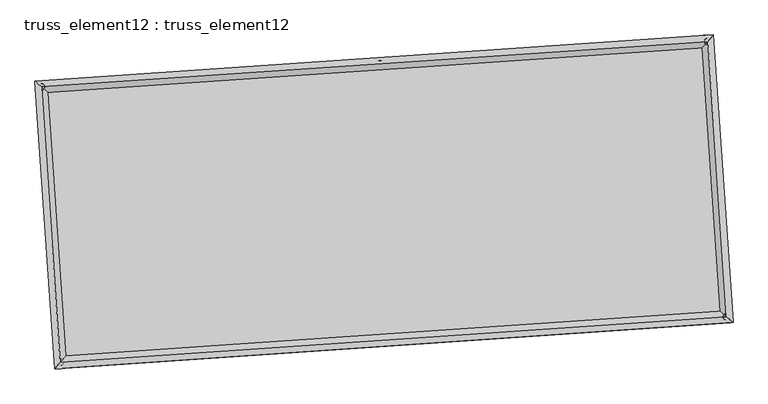
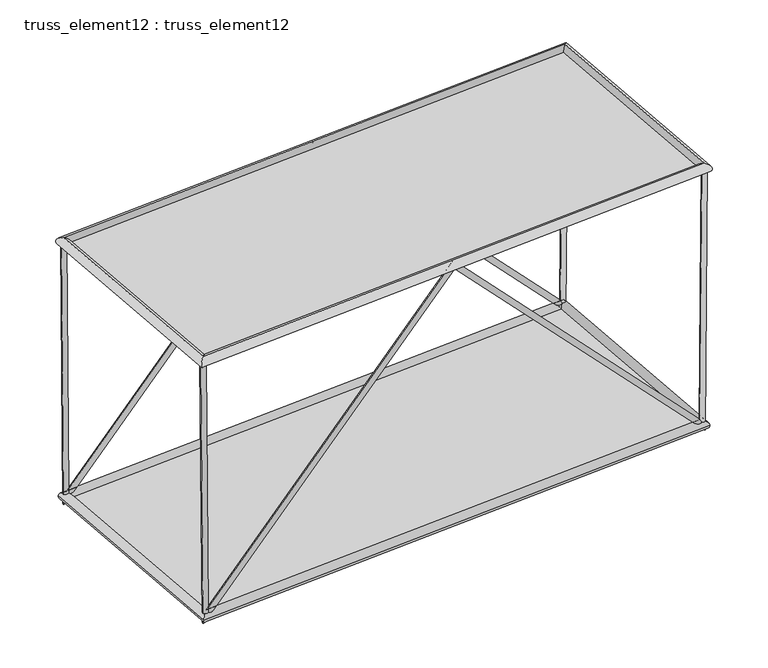
"""IFC4 building model written with IfcOpenShell, lengths in millimetres: plate geometry, truss_element12 : truss_element12."""

from ifc_helpers import new_model, si_unit, frame, origin, origin_with_axes, place, context, project, spatial, polyline, circle_curve, ellipse_curve, outline, extrude, source, transform, mapped, element, save
from ifc_brep_helpers import plane_surface, cylinder_surface, advanced_brep


def truss_element12_truss_element12_5f5549ff(model_context):
    return source(origin(), model_context, "Body", "SolidModel", [
        advanced_brep(
        [(-3707.9964238, 2273.2882323, 5000.2443705), (-3807.096081, 2259.9272328, 4999.3831901), (-3665.9998224, 2276.1518209, 123.0904436), (-3762.9870604, 2262.9348592, -123.0904436), (1064.0881488, 2598.6785389, 5071.9331188), (1064.5308451, 2592.1049541, 4927.688056), (5793.4565797, 2921.1561942, 123.0852691), (5891.3043973, 2921.2242943, -123.0852691), (5836.1672791, 2924.0684744, 5000.2453052), (5936.1632135, 2924.2830465, 4999.3694838)],
        [
            (0, 1, circle_curve(frame((-3757.5462524, 2266.6077325, 4999.8137803), z_axis=(-0.008610562197328881, -0.0005871215044246289, 0.9999627560599369), x_axis=(-0.13361007490078702, 0.9910338160498287, -0.0005686217728233661)), 50.0)),
            (1, 0, circle_curve(frame((-3757.5462524, 2266.6077325, 4999.8137803), z_axis=(-0.008610562197328881, -0.0005871215044246289, 0.9999627560599369), x_axis=(-0.13361007490078702, 0.9910338160498287, -0.0005686217728233661)), 50.0)),
            (0, 2),
            (2, 3, ellipse_curve(frame((-3714.4934414, 2269.54334, 0.0), z_axis=(-0.9273750844968209, -0.06323418172910877, 0.3687504453089708), x_axis=(0.36789619657997696, 0.02508544314041891, 0.9295284337148788)), 132.7108104, 50.0)),
            (3, 1),
            (3, 2, ellipse_curve(frame((-3714.4934414, 2269.54334, 0.0), z_axis=(-0.9273750844968209, -0.06323418172910877, 0.3687504453089708), x_axis=(0.36789619657997696, 0.02508544314041891, 0.9295284337148788)), 132.7108104, 50.0)),
            (2, 4),
            (4, 5, ellipse_curve(frame((1064.309497, 2595.3917465, 4999.8105874), z_axis=(-0.9976833953446986, -0.06802823817891461, 3.825893912910826e-05), x_axis=(-3.817030832084868e-05, -2.6026882256253026e-06, -0.9999999992681269)), 72.2795775, 50.0)),
            (5, 3),
            (5, 4, ellipse_curve(frame((1064.309497, 2595.3917465, 4999.8105874), z_axis=(-0.9976833953446986, -0.06802823817891461, 3.825893912910826e-05), x_axis=(-3.817030832084868e-05, -2.6026882256253026e-06, -0.9999999992681269)), 72.2795775, 50.0)),
            (4, 6),
            (6, 7, ellipse_curve(frame((5842.3804885, 2921.1902443, 0.0), z_axis=(-0.9274161456323363, -0.06323698153185128, -0.3686466831360366), x_axis=(-0.3677926747828999, -0.025078384382599298, 0.9295695901936544)), 132.6993561, 50.0)),
            (7, 5),
            (7, 6, ellipse_curve(frame((5842.3804885, 2921.1902443, 0.0), z_axis=(-0.9274161456323363, -0.06323698153185128, -0.3686466831360366), x_axis=(-0.3677926747828999, -0.025078384382599298, 0.9295695901936544)), 132.6993561, 50.0)),
            (8, 9, circle_curve(frame((5886.1652463, 2924.1757604, 4999.8073945), z_axis=(0.00875695156738284, 0.0005971032390905219, 0.9999614788915463), x_axis=(-0.002150867604689313, 0.9999975196721189, -0.0005782889909695317)), 50.0)),
            (9, 8, circle_curve(frame((5886.1652463, 2924.1757604, 4999.8073945), z_axis=(0.00875695156738284, 0.0005971032390905219, 0.9999614788915463), x_axis=(-0.002150867604689313, 0.9999975196721189, -0.0005782889909695317)), 50.0)),
            (6, 8),
            (9, 7),
        ],
        [
            plane_surface(frame((-3757.5462524, 2316.6077239, 4999.8431375), z_axis=(-0.008610562197328035, -0.0005871215044280537, 0.9999627560599371), x_axis=(0.999962928422172, -5.055633651274154e-06, 0.008610560713137268))),
            cylinder_surface(frame((-3757.5462524, 2266.6077325, 4999.8137803), z_axis=(-0.008610562197328883, -0.000587121504424629, 0.9999627560599371), x_axis=(-0.13361007490078702, 0.9910338160498287, -0.0005686217728233661)), 50.0),
            cylinder_surface(frame((-3714.4934414, 2269.54334, 0.0), z_axis=(-0.6901833653788351, -0.04706098005258923, -0.7221026148068121), x_axis=(-0.02041511250677689, 0.9987521502411405, -0.04557812600397415)), 50.0),
            cylinder_surface(frame((1064.309497, 2595.3917465, 4999.8105874), z_axis=(-0.6901282375994761, -0.047057221098874814, 0.7221555466866489), x_axis=(-0.11534922537103473, 0.9922789539632748, -0.045574485491901566)), 50.0),
            plane_surface(frame((5886.1652463, 2874.1757694, 4999.8372508), z_axis=(0.00875695156738239, 0.0005971032390901972, 0.9999614788915465), x_axis=(0.9999616571645369, -5.2290046408387525e-06, -0.008756950006194586))),
            cylinder_surface(frame((5842.3804885, 2921.1902443, 0.0), z_axis=(-0.00875695156738284, -0.0005971032390905219, -0.9999614788915463), x_axis=(-0.002150867604689313, 0.9999975196721189, -0.0005782889909695317)), 50.0),
        ],
        [
            (0, [[1, 2]]),
            (1, [[-1, 3, 4, 5]]),
            (1, [[-2, -5, 6, -3]]),
            (2, [[-4, 7, 8, 9]]),
            (2, [[-6, -9, 10, -7]]),
            (3, [[-8, 11, 12, 13]]),
            (3, [[-10, -13, 14, -11]]),
            (4, [[15, 16]]),
            (5, [[-12, 17, -16, 18]]),
            (5, [[-14, -18, -15, -17]]),
        ],
    ),
        advanced_brep(
        [(-3435.8834709, -1717.445352, 5000.2443705), (-3534.9831281, -1730.8063515, 4999.3831901), (-3393.8868695, -1714.5817634, 123.0904436), (-3490.8741075, -1727.7987251, -123.0904436), (1336.2011017, -1392.0550454, 5071.9331188), (1336.643798, -1398.6286302, 4927.688056), (6065.5695326, -1069.5773901, 123.0852691), (6163.4173503, -1069.50929, -123.0852691), (6108.2802321, -1066.6651099, 5000.2453052), (6208.2761665, -1066.4505378, 4999.3694838)],
        [
            (0, 1, circle_curve(frame((-3485.4332995, -1724.1258518, 4999.8137803), z_axis=(-0.008610562197328883, -0.0005871215044246118, 0.9999627560599369), x_axis=(-0.13361007490078664, 0.9910338160498287, -0.0005686217728233801)), 50.0)),
            (1, 0, circle_curve(frame((-3485.4332995, -1724.1258518, 4999.8137803), z_axis=(-0.008610562197328883, -0.0005871215044246118, 0.9999627560599369), x_axis=(-0.13361007490078664, 0.9910338160498287, -0.0005686217728233801)), 50.0)),
            (0, 2),
            (2, 3, ellipse_curve(frame((-3442.3804885, -1721.1902443, 0.0), z_axis=(-0.9273750844968209, -0.06323418172910855, 0.3687504453089707), x_axis=(0.3678961965799769, 0.025085443140418835, 0.9295284337148788)), 132.7108104, 50.0)),
            (3, 1),
            (3, 2, ellipse_curve(frame((-3442.3804885, -1721.1902443, 0.0), z_axis=(-0.9273750844968209, -0.06323418172910855, 0.3687504453089707), x_axis=(0.3678961965799769, 0.025085443140418835, 0.9295284337148788)), 132.7108104, 50.0)),
            (2, 4),
            (4, 5, ellipse_curve(frame((1336.4224499, -1395.3418378, 4999.8105874), z_axis=(-0.9976833953446986, -0.06802823817891454, 3.825893912894776e-05), x_axis=(-3.817030832069493e-05, -2.6026882254811685e-06, -0.9999999992681269)), 72.2795775, 50.0)),
            (5, 3),
            (5, 4, ellipse_curve(frame((1336.4224499, -1395.3418378, 4999.8105874), z_axis=(-0.9976833953446986, -0.06802823817891454, 3.825893912894776e-05), x_axis=(-3.817030832069493e-05, -2.6026882254811685e-06, -0.9999999992681269)), 72.2795775, 50.0)),
            (4, 6),
            (6, 7, ellipse_curve(frame((6114.4934414, -1069.54334, 0.0), z_axis=(-0.9274161456323362, -0.06323698153185144, -0.3686466831360369), x_axis=(-0.36779267478290023, -0.025078384382599305, 0.9295695901936543)), 132.6993561, 50.0)),
            (7, 5),
            (7, 6, ellipse_curve(frame((6114.4934414, -1069.54334, 0.0), z_axis=(-0.9274161456323362, -0.06323698153185144, -0.3686466831360369), x_axis=(-0.36779267478290023, -0.025078384382599305, 0.9295695901936543)), 132.6993561, 50.0)),
            (8, 9, circle_curve(frame((6158.2781993, -1066.5578239, 4999.8073945), z_axis=(0.00875695156738245, 0.0005971032390905659, 0.9999614788915463), x_axis=(-0.002150867604689674, 0.999997519672119, -0.0005782889909695735)), 50.0)),
            (9, 8, circle_curve(frame((6158.2781993, -1066.5578239, 4999.8073945), z_axis=(0.00875695156738245, 0.0005971032390905659, 0.9999614788915463), x_axis=(-0.002150867604689674, 0.999997519672119, -0.0005782889909695735)), 50.0)),
            (6, 8),
            (9, 7),
        ],
        [
            plane_surface(frame((-3485.4332995, -1674.1258604, 4999.8431375), z_axis=(-0.008610562197328035, -0.0005871215044280489, 0.9999627560599371), x_axis=(0.999962928422172, -5.055633651274154e-06, 0.008610560713137268))),
            cylinder_surface(frame((-3485.4332995, -1724.1258518, 4999.8137803), z_axis=(-0.008610562197328885, -0.0005871215044246119, 0.9999627560599371), x_axis=(-0.13361007490078664, 0.9910338160498287, -0.0005686217728233801)), 50.0),
            cylinder_surface(frame((-3442.3804885, -1721.1902443, 0.0), z_axis=(-0.690183365378835, -0.047060980052589074, -0.7221026148068123), x_axis=(-0.02041511250677676, 0.9987521502411404, -0.045578126003974054)), 50.0),
            cylinder_surface(frame((1336.4224499, -1395.3418378, 4999.8105874), z_axis=(-0.6901282375994762, -0.04705722109887487, 0.7221555466866488), x_axis=(-0.11534922537103474, 0.9922789539632748, -0.045574485491901524)), 50.0),
            plane_surface(frame((6158.2781993, -1116.5578149, 4999.8372508), z_axis=(0.00875695156738239, 0.0005971032390901939, 0.9999614788915465), x_axis=(0.9999616571645369, -5.229004640394663e-06, -0.008756950006194586))),
            cylinder_surface(frame((6114.4934414, -1069.54334, 0.0), z_axis=(-0.00875695156738245, -0.0005971032390905659, -0.9999614788915463), x_axis=(-0.002150867604689674, 0.999997519672119, -0.0005782889909695735)), 50.0),
        ],
        [
            (0, [[1, 2]]),
            (1, [[-1, 3, 4, 5]]),
            (1, [[-2, -5, 6, -3]]),
            (2, [[-4, 7, 8, 9]]),
            (2, [[-6, -9, 10, -7]]),
            (3, [[-8, 11, 12, 13]]),
            (3, [[-10, -13, 14, -11]]),
            (4, [[15, 16]]),
            (5, [[-12, 17, -16, 18]]),
            (5, [[-14, -18, -15, -17]]),
        ],
    ),
        advanced_brep(
        [(-3485.434982, -1724.1277166, 4909.8137803), (-3485.431617, -1724.123987, 5089.8137803), (-3757.5443323, 2266.6061134, 5089.8137803), (-3757.5481725, 2266.6093517, 4909.8137803), (5886.1636825, 2924.1739037, 5089.8073944), (5886.1668102, 2924.1776171, 4909.8073945), (6158.2763978, -1066.5561966, 5089.8073944), (6158.2800007, -1066.5594511, 4909.8073945)],
        [
            (0, 1, ellipse_curve(frame((-3485.4332995, -1724.1258518, 4999.8137803), z_axis=(-0.7535719234053024, 0.6573654662780931, 4.6714499693675804e-07), x_axis=(-0.6573654662779286, -0.753571923405446, 4.6714499693680886e-07)), 127.2792206, 90.0)),
            (1, 2),
            (2, 3, ellipse_curve(frame((-3757.5462524, 2266.6077325, 4999.8137803), z_axis=(-0.6573654662779286, -0.753571923405446, 4.6714499693685635e-07), x_axis=(0.7535719234053025, -0.657365466278093, -4.6714499693680563e-07)), 127.2792206, 90.0)),
            (3, 0),
            (1, 0, ellipse_curve(frame((-3485.4332995, -1724.1258518, 4999.8137803), z_axis=(-0.7535719234053024, 0.6573654662780931, 4.6714499693675804e-07), x_axis=(-0.6573654662779286, -0.753571923405446, 4.6714499693680886e-07)), 127.2792206, 90.0)),
            (3, 2, ellipse_curve(frame((-3757.5462524, 2266.6077325, 4999.8137803), z_axis=(-0.6573654662779286, -0.753571923405446, 4.6714499693685635e-07), x_axis=(0.7535719234053025, -0.657365466278093, -4.6714499693680563e-07)), 127.2792206, 90.0)),
            (2, 4),
            (4, 5, ellipse_curve(frame((5886.1652463, 2924.1757604, 4999.8073945), z_axis=(-0.7535719234053022, 0.6573654662780931, 4.671449969368529e-07), x_axis=(-0.657365466277929, -0.7535719234054455, 4.6714499693680907e-07)), 127.2792206, 90.0)),
            (5, 3),
            (5, 4, ellipse_curve(frame((5886.1652463, 2924.1757604, 4999.8073945), z_axis=(-0.7535719234053022, 0.6573654662780931, 4.671449969368529e-07), x_axis=(-0.657365466277929, -0.7535719234054455, 4.6714499693680907e-07)), 127.2792206, 90.0)),
            (4, 6),
            (6, 7, ellipse_curve(frame((6158.2781993, -1066.5578239, 4999.8073945), z_axis=(0.6573654662779289, 0.7535719234054455, -4.671449969367615e-07), x_axis=(-0.7535719234053019, 0.6573654662780936, 4.671449969368051e-07)), 127.2792206, 90.0)),
            (7, 5),
            (7, 6, ellipse_curve(frame((6158.2781993, -1066.5578239, 4999.8073945), z_axis=(0.6573654662779289, 0.7535719234054455, -4.671449969367615e-07), x_axis=(-0.7535719234053019, 0.6573654662780936, 4.671449969368051e-07)), 127.2792206, 90.0)),
            (6, 1),
            (0, 7),
        ],
        [
            cylinder_surface(frame((-3485.4332995, -1724.1258518, 4999.8137803), z_axis=(0.06802823822869912, -0.9976833960748768, 0.0), x_axis=(-0.997683395874126, -0.0680282382150107, 2.0060750261440357e-05)), 90.0),
            cylinder_surface(frame((-3757.5462524, 2266.6077325, 4999.8137803), z_axis=(-0.9976833960746592, -0.06802823822868387, 6.606427902628043e-07), x_axis=(-0.06802823820311017, 0.9976833958880026, 1.9400107471301905e-05)), 90.0),
            cylinder_surface(frame((5886.1652463, 2924.1757604, 4999.8073945), z_axis=(-0.06802823822869865, 0.997683396074877, 0.0), x_axis=(0.9976833958996999, 0.068028238216754, 1.873946468116346e-05)), 90.0),
            cylinder_surface(frame((6158.2781993, -1066.5578239, 4999.8073945), z_axis=(0.9976833960746592, 0.06802823822868365, -6.606427902627372e-07), x_axis=(0.06802823822868365, -0.9976833958862589, 1.9400107471301912e-05)), 90.0),
        ],
        [
            (0, [[1, 2, 3, 4]]),
            (0, [[5, -4, 6, -2]]),
            (1, [[-3, 7, 8, 9]]),
            (1, [[-6, -9, 10, -7]]),
            (2, [[-8, 11, 12, 13]]),
            (2, [[-10, -13, 14, -11]]),
            (3, [[-12, 15, -1, 16]]),
            (3, [[-14, -16, -5, -15]]),
        ],
    ),
        advanced_brep(
        [(-3358.7115243, -1625.2761972, 0.0), (-3526.0494527, -1817.1042913, 0.0), (-3810.4074885, 2353.2123043, 0.0), (-3618.5793943, 2185.8743758, 0.0), (5926.0494527, 3017.1042913, 0.0), (5758.7115243, 2825.2761972, 0.0), (6210.4074885, -1153.2123043, 0.0), (6018.5793943, -985.8743758, 0.0)],
        [
            (0, 1, ellipse_curve(frame((-3442.3804885, -1721.1902443, 0.0), z_axis=(-0.753571923405459, 0.6573654662780796, 0.0), x_axis=(-0.6573654662780796, -0.753571923405459, 0.0)), 127.2792206, 90.0)),
            (1, 2),
            (2, 3, ellipse_curve(frame((-3714.4934414, 2269.54334, 0.0), z_axis=(-0.6573654662780796, -0.753571923405459, 0.0), x_axis=(0.753571923405459, -0.6573654662780796, 0.0)), 127.2792206, 90.0)),
            (3, 0),
            (1, 0, ellipse_curve(frame((-3442.3804885, -1721.1902443, 0.0), z_axis=(-0.753571923405459, 0.6573654662780796, 0.0), x_axis=(-0.6573654662780796, -0.753571923405459, 0.0)), 127.2792206, 90.0)),
            (3, 2, ellipse_curve(frame((-3714.4934414, 2269.54334, 0.0), z_axis=(-0.6573654662780796, -0.753571923405459, 0.0), x_axis=(0.753571923405459, -0.6573654662780796, 0.0)), 127.2792206, 90.0)),
            (2, 4),
            (4, 5, ellipse_curve(frame((5842.3804885, 2921.1902443, 0.0), z_axis=(-0.7535719234054589, 0.6573654662780797, 0.0), x_axis=(-0.6573654662780798, -0.7535719234054588, 0.0)), 127.2792206, 90.0)),
            (5, 3),
            (5, 4, ellipse_curve(frame((5842.3804885, 2921.1902443, 0.0), z_axis=(-0.7535719234054589, 0.6573654662780797, 0.0), x_axis=(-0.6573654662780798, -0.7535719234054588, 0.0)), 127.2792206, 90.0)),
            (4, 6),
            (6, 7, ellipse_curve(frame((6114.4934414, -1069.54334, 0.0), z_axis=(0.6573654662780797, 0.7535719234054589, 0.0), x_axis=(-0.7535719234054589, 0.6573654662780798, 0.0)), 127.2792206, 90.0)),
            (7, 5),
            (7, 6, ellipse_curve(frame((6114.4934414, -1069.54334, 0.0), z_axis=(0.6573654662780797, 0.7535719234054589, 0.0), x_axis=(-0.7535719234054589, 0.6573654662780798, 0.0)), 127.2792206, 90.0)),
            (6, 1),
            (0, 7),
        ],
        [
            cylinder_surface(frame((-3442.3804885, -1721.1902443, 0.0), z_axis=(0.06802823822870309, -0.9976833960748764, 0.0), x_axis=(-0.9976833960748764, -0.06802823822870309, 0.0)), 90.0),
            cylinder_surface(frame((-3714.4934414, 2269.54334, 0.0), z_axis=(-0.9976833960748764, -0.06802823822870262, 0.0), x_axis=(-0.06802823822870262, 0.9976833960748764, 0.0)), 90.0),
            cylinder_surface(frame((5842.3804885, 2921.1902443, 0.0), z_axis=(-0.06802823822870294, 0.9976833960748767, 0.0), x_axis=(0.9976833960748767, 0.06802823822870294, 0.0)), 90.0),
            cylinder_surface(frame((6114.4934414, -1069.54334, 0.0), z_axis=(0.9976833960748767, 0.06802823822870246, 0.0), x_axis=(0.06802823822870246, -0.9976833960748767, 0.0)), 90.0),
        ],
        [
            (0, [[1, 2, 3, 4]]),
            (0, [[5, -4, 6, -2]]),
            (1, [[-3, 7, 8, 9]]),
            (1, [[-6, -9, 10, -7]]),
            (2, [[-8, 11, 12, 13]]),
            (2, [[-10, -13, 14, -11]]),
            (3, [[-12, 15, -1, 16]]),
            (3, [[-14, -16, -5, -15]]),
        ],
    ),
        extrude(outline(polyline([(-3442.3804885, -1721.1902443), (-3714.4934414, 2269.54334), (5842.3804885, 2921.1902443), (6114.4934414, -1069.54334), (-3442.3804885, -1721.1902443)])), origin_with_axes(), (0.0, 0.0, 1.0), 20.0),
        extrude(outline(polyline([(-2000.0, 4833.0520166), (2000.0, 4833.0520166), (2000.0, -4833.0520166), (-2000.0, -4833.0520167), (-2000.0, 4833.0520166)])), frame((1200.3659734, 600.0249543, 4999.8105874), z_axis=(6.591123425817434e-07, 4.494236512007069e-08, 0.9999999999997817), x_axis=(-0.0680282382287028, 0.9976833960748765, 0.0)), (0.0, 0.0, 1.0), 20.0),
    ])


if __name__ == "__main__":
    model = new_model("IFC4")
    model_context = context("Model", 3, world=origin())
    ifc_project = project(units=[si_unit("LENGTHUNIT", "METRE", prefix="MILLI")], contexts=[model_context])
    site = spatial("IfcSite", under=ifc_project)
    building = spatial("IfcBuilding", under=site)
    placement = place(None, origin())
    truss_element12_truss_element12_shape = truss_element12_truss_element12_5f5549ff(model_context)
    element("IfcPlate", 1, ObjectType="truss_element12 : truss_element12", at=placement, inside=building, context=model_context, shape_type="MappedRepresentation", body=[
        mapped(truss_element12_truss_element12_shape, transform((0.0, 0.0, 0.0), x_axis=(1.0, 0.0, 0.0), y_axis=(0.0, 1.0, 0.0), z_axis=(0.0, 0.0, 1.0))),
    ])
    save(model, "model.ifc")

# Revit data of these elements
# Type "truss_element12 : truss_element12"
#   steellbar1 = 90 mm
#   steelbar2 = 50 mm
#   offset1 = 5000 mm
#   M = Default Roof
# Element 1 (IfcPlate, "truss_element12 : truss_element12")
#   Materials on its faces: "Default Roof"
# Materials
#   "Default Roof": class "Miscellaneous", colour RGB 0 127 0, transparency 0, Comments = "Rendering appearance not upgraded Rendering appearance not upgraded ", Cost = 0
